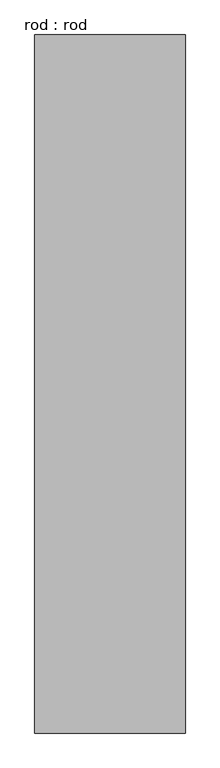
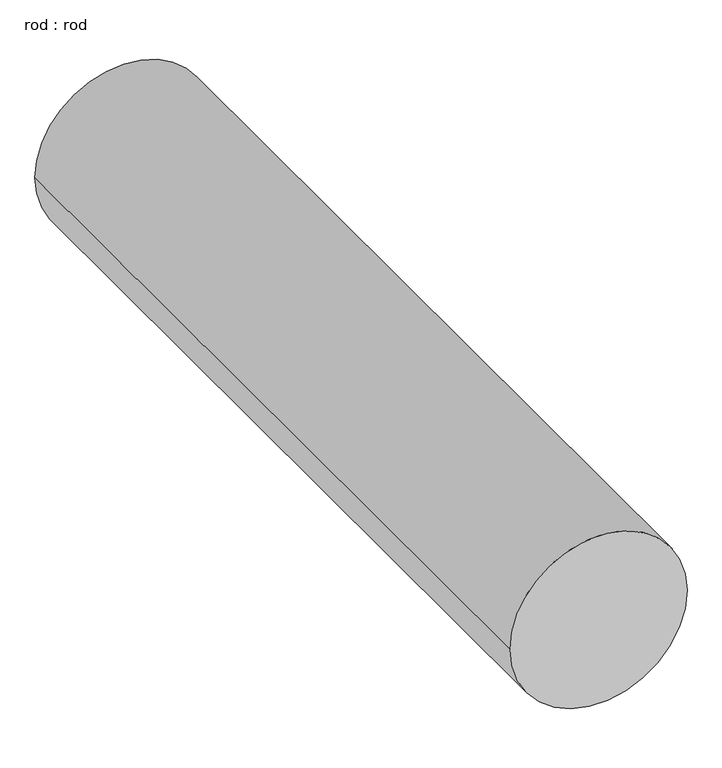
"""IFC4 building model written with IfcOpenShell, lengths in millimetres: proxy geometry, rod : rod."""

from ifc_helpers import new_model, si_unit, point, frame, frame_2d, origin, place, context, project, spatial, circle_curve, trimmed, segment, composite_curve, outline, extrude, source, transform, mapped, element, save


def rod_rod_061603c3(model_context):
    return source(origin(), model_context, "Body", "SweptSolid", [
        extrude(outline(composite_curve([segment(trimmed(circle_curve(frame_2d((0.0108462, 0.0)), 200.0), [point((0.0108462, 200.0))], [point((0.0108462, -200.0))], False, "CARTESIAN"), True, "CONTINUOUS"), segment(trimmed(circle_curve(frame_2d((0.0108462, 0.0)), 200.0), [point((0.0108462, -200.0))], [point((0.0108462, 200.0))], False, "CARTESIAN"), True, "CONTINUOUS")], self_intersect=False)), frame((0.0, 3165.6060506, 0.0), z_axis=(0.0, 1.0, 0.0), x_axis=(0.0, 0.0, 1.0)), (0.0, 0.0, 1.0), 1854.2451294),
    ])


if __name__ == "__main__":
    model = new_model("IFC4")
    model_context = context("Model", 3, world=origin())
    ifc_project = project(units=[si_unit("LENGTHUNIT", "METRE", prefix="MILLI")], contexts=[model_context])
    site = spatial("IfcSite", under=ifc_project)
    building = spatial("IfcBuilding", under=site)
    placement = place(None, origin())
    rod_rod_shape = rod_rod_061603c3(model_context)
    element("IfcBuildingElementProxy", 1, Name="rod : rod", ObjectType="rod : rod", at=placement, inside=building, context=model_context, shape_type="MappedRepresentation", body=[
        mapped(rod_rod_shape, transform((0.0, 0.0, 0.0), x_axis=(1.0, 0.0, 0.0), y_axis=(0.0, 1.0, 0.0), z_axis=(0.0, 0.0, 1.0))),
    ])
    save(model, "model.ifc")

# Revit data of these elements
# Type "rod : rod"
#   Default Elevation = 0
